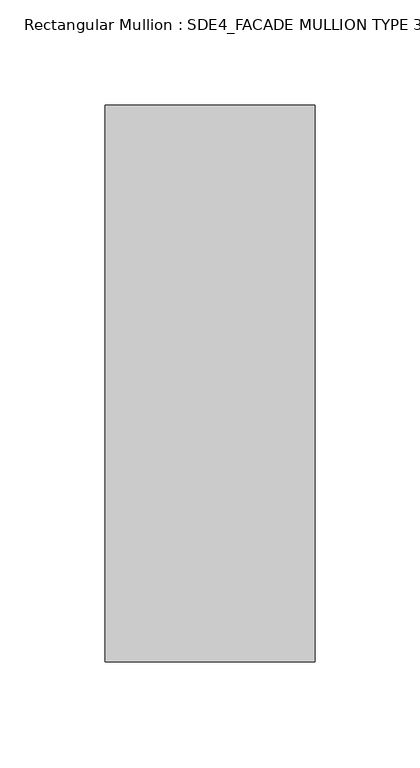
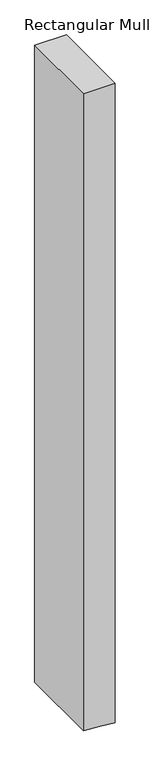
"""IFC4 building model written with IfcOpenShell, lengths in millimetres: member geometry, Rectangular Mullion : SDE4_FACADE MULLION TYPE 3."""

from ifc_helpers import new_model, si_unit, frame, origin, place, context, project, spatial, polyline, outline, extrude, source, transform, mapped, element, save


def rectangular_mullion_sde4_facade_mullion_type_3_f6a6c305(model_context):
    return source(origin(), model_context, "Body", "SweptSolid", [
        extrude(outline(polyline([(0.0, 50.0), (0.0, -50.0), (-2119.5195266, -50.0), (-2123.5856057, 3.056508), (-2127.183203, 50.0), (0.0, 50.0)])), frame((0.0, -132.5, 0.0), z_axis=(0.0, 1.0, 0.0), x_axis=(0.0, 0.0, 1.0)), (0.0, 0.0, 1.0), 265.0),
    ])


if __name__ == "__main__":
    model = new_model("IFC4")
    model_context = context("Model", 3, world=origin())
    ifc_project = project(units=[si_unit("LENGTHUNIT", "METRE", prefix="MILLI")], contexts=[model_context])
    site = spatial("IfcSite", under=ifc_project)
    building = spatial("IfcBuilding", under=site)
    placement = place(None, origin())
    rectangular_mullion_sde4_facade_mullion_type_3_shape = rectangular_mullion_sde4_facade_mullion_type_3_f6a6c305(model_context)
    element("IfcMember", 1, ObjectType="Rectangular Mullion : SDE4_FACADE MULLION TYPE 3", at=placement, inside=building, context=model_context, shape_type="MappedRepresentation", body=[
        mapped(rectangular_mullion_sde4_facade_mullion_type_3_shape, transform((0.0, 0.0, 0.0), x_axis=(1.0, 0.0, 0.0), y_axis=(0.0, 1.0, 0.0), z_axis=(0.0, 0.0, 1.0))),
    ])
    save(model, "model.ifc")

# Revit data of these elements
# Type "Rectangular Mullion : SDE4_FACADE MULLION TYPE 3"
#   built-in parameter 1007322 = 0.869423 (stored number, unit not read)
#   built-in parameter 1007321 = 0.164042 (stored number, unit not read)
#   built-in parameter 1007320 = 0.164042 (stored number, unit not read)
